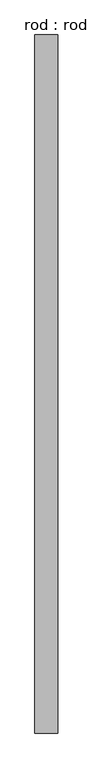
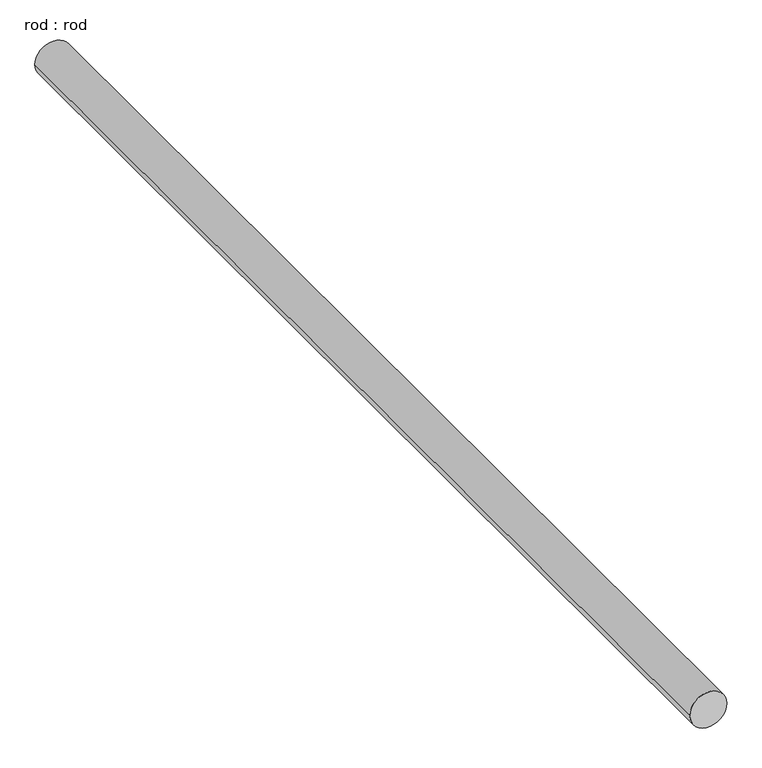
"""IFC4 building model written with IfcOpenShell, lengths in millimetres: proxy geometry, rod : rod."""

from ifc_helpers import new_model, si_unit, point, frame, frame_2d, origin, place, context, project, spatial, circle_curve, trimmed, segment, composite_curve, outline, extrude, source, transform, mapped, element, save


def rod_rod_55220521(model_context):
    return source(origin(), model_context, "Body", "SweptSolid", [
        extrude(outline(composite_curve([segment(trimmed(circle_curve(frame_2d((0.0108462, 0.0)), 200.0), [point((0.0108462, 200.0))], [point((0.0108462, -200.0))], False, "CARTESIAN"), True, "CONTINUOUS"), segment(trimmed(circle_curve(frame_2d((0.0108462, 0.0)), 200.0), [point((0.0108462, -200.0))], [point((0.0108462, 200.0))], False, "CARTESIAN"), True, "CONTINUOUS")], self_intersect=False)), frame((0.0, -2048.4622469, 0.0), z_axis=(0.0, 1.0, 0.0), x_axis=(0.0, 0.0, 1.0)), (0.0, 0.0, 1.0), 12282.3817245),
    ])


if __name__ == "__main__":
    model = new_model("IFC4")
    model_context = context("Model", 3, world=origin())
    ifc_project = project(units=[si_unit("LENGTHUNIT", "METRE", prefix="MILLI")], contexts=[model_context])
    site = spatial("IfcSite", under=ifc_project)
    building = spatial("IfcBuilding", under=site)
    placement = place(None, origin())
    rod_rod_shape = rod_rod_55220521(model_context)
    element("IfcBuildingElementProxy", 1, Name="rod : rod", ObjectType="rod : rod", at=placement, inside=building, context=model_context, shape_type="MappedRepresentation", body=[
        mapped(rod_rod_shape, transform((0.0, 0.0, 0.0), x_axis=(1.0, 0.0, 0.0), y_axis=(0.0, 1.0, 0.0), z_axis=(0.0, 0.0, 1.0))),
    ])
    save(model, "model.ifc")

# Revit data of these elements
# Type "rod : rod"
#   Default Elevation = 0
